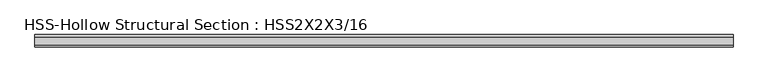
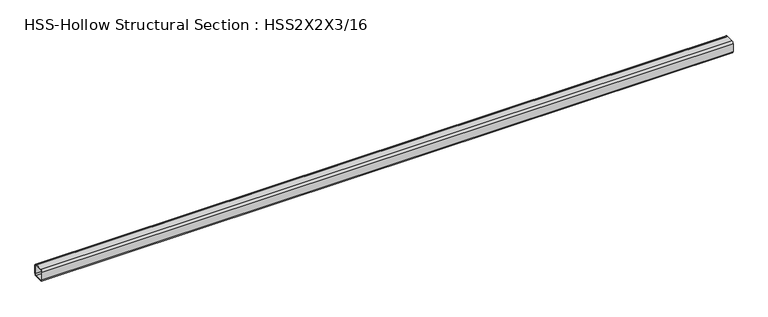
"""IFC4 building model written with IfcOpenShell, lengths in millimetres: beam geometry, HSS-Hollow Structural Section : HSS2X2X3/16."""

from ifc_helpers import new_model, si_unit, point, frame, frame_2d, origin, place, context, project, spatial, polyline, circle_curve, trimmed, segment, composite_curve, outline, extrude, source, transform, mapped, element, save


def hss_hollow_structural_section_hss2x2x3_16_75d81287(model_context):
    return source(origin(), model_context, "Body", "SweptSolid", [
        extrude(outline(composite_curve([segment(polyline([(25.4, 16.5608), (25.4, -16.5608)]), True, "CONTINUOUS"), segment(trimmed(circle_curve(frame_2d((16.5608, -16.5608)), 8.8392), [point((25.4, -16.5608))], [point((16.5608, -25.4))], False, "CARTESIAN"), True, "CONTINUOUS"), segment(polyline([(16.5608, -25.4), (-16.5608, -25.4)]), True, "CONTINUOUS"), segment(trimmed(circle_curve(frame_2d((-16.5608, -16.5608)), 8.8392), [point((-16.5608, -25.4))], [point((-25.4, -16.5608))], False, "CARTESIAN"), True, "CONTINUOUS"), segment(polyline([(-25.4, -16.5608), (-25.4, 16.5608)]), True, "CONTINUOUS"), segment(trimmed(circle_curve(frame_2d((-16.5608, 16.5608)), 8.8392), [point((-25.4, 16.5608))], [point((-16.5608, 25.4))], False, "CARTESIAN"), True, "CONTINUOUS"), segment(polyline([(-16.5608, 25.4), (16.5608, 25.4)]), True, "CONTINUOUS"), segment(trimmed(circle_curve(frame_2d((16.5608, 16.5608)), 8.8392), [point((16.5608, 25.4))], [point((25.4, 16.5608))], False, "CARTESIAN"), True, "CONTINUOUS")], self_intersect=False), holes=[composite_curve([segment(trimmed(circle_curve(frame_2d((-16.5608, 16.5608)), 4.4196), [point((-16.5608, 20.9804))], [point((-20.9804, 16.5608))], True, "CARTESIAN"), True, "CONTINUOUS"), segment(polyline([(-20.9804, 16.5608), (-20.9804, -16.5608)]), True, "CONTINUOUS"), segment(trimmed(circle_curve(frame_2d((-16.5608, -16.5608)), 4.4196), [point((-20.9804, -16.5608))], [point((-16.5608, -20.9804))], True, "CARTESIAN"), True, "CONTINUOUS"), segment(polyline([(-16.5608, -20.9804), (16.5608, -20.9804)]), True, "CONTINUOUS"), segment(trimmed(circle_curve(frame_2d((16.5608, -16.5608)), 4.4196), [point((16.5608, -20.9804))], [point((20.9804, -16.5608))], True, "CARTESIAN"), True, "CONTINUOUS"), segment(polyline([(20.9804, -16.5608), (20.9804, 16.5608)]), True, "CONTINUOUS"), segment(trimmed(circle_curve(frame_2d((16.5608, 16.5608)), 4.4196), [point((20.9804, 16.5608))], [point((16.5608, 20.9804))], True, "CARTESIAN"), True, "CONTINUOUS"), segment(polyline([(16.5608, 20.9804), (-16.5608, 20.9804)]), True, "CONTINUOUS")], self_intersect=False)]), frame((-533.4, 0.0, 0.0), z_axis=(1.0, 0.0, 0.0), x_axis=(0.0, 1.0, 0.0)), (0.0, 0.0, 1.0), 2860.0936767),
    ])


if __name__ == "__main__":
    model = new_model("IFC4")
    model_context = context("Model", 3, world=origin())
    ifc_project = project(units=[si_unit("LENGTHUNIT", "METRE", prefix="MILLI")], contexts=[model_context])
    site = spatial("IfcSite", under=ifc_project)
    building = spatial("IfcBuilding", under=site)
    placement = place(None, origin())
    hss_hollow_structural_section_hss2x2x3_16_shape = hss_hollow_structural_section_hss2x2x3_16_75d81287(model_context)
    element("IfcBeam", 1, ObjectType="HSS-Hollow Structural Section : HSS2X2X3/16", at=placement, inside=building, context=model_context, shape_type="MappedRepresentation", body=[
        mapped(hss_hollow_structural_section_hss2x2x3_16_shape, transform((0.0, 0.0, 0.0), x_axis=(1.0, 0.0, 0.0), y_axis=(0.0, 1.0, 0.0), z_axis=(0.0, 0.0, 1.0))),
    ])
    save(model, "model.ifc")

# Revit data of these elements
# Type "HSS-Hollow Structural Section : HSS2X2X3/16"
#   Assembly Code = "B10"
#   Shape = "Square"
#   W = 4.3
#   Ht = 0' - 2"
#   Length [instance default] = 5' - 0"
#   b = 0' - 2"
#   kr = 0' - 0.348"
#   t = 0' - 0.174"
#   A = 0.00826389 SF
#   Structural Material [instance default] = none
# Element 1 (IfcBeam, "HSS-Hollow Structural Section : HSS2X2X3/16")
#   Structural Material = _STRUCTURAL STEEL (SEE STRUCT. DWGS)
#   Materials on its faces: "_STRUCTURAL STEEL (SEE STRUCT. DWGS)"
# Materials
#   "_STRUCTURAL STEEL (SEE STRUCT. DWGS)": class "Metal", colour RGB 199 199 199, transparency 0, Description = "Structural steel 50ksi", Cost = 0
